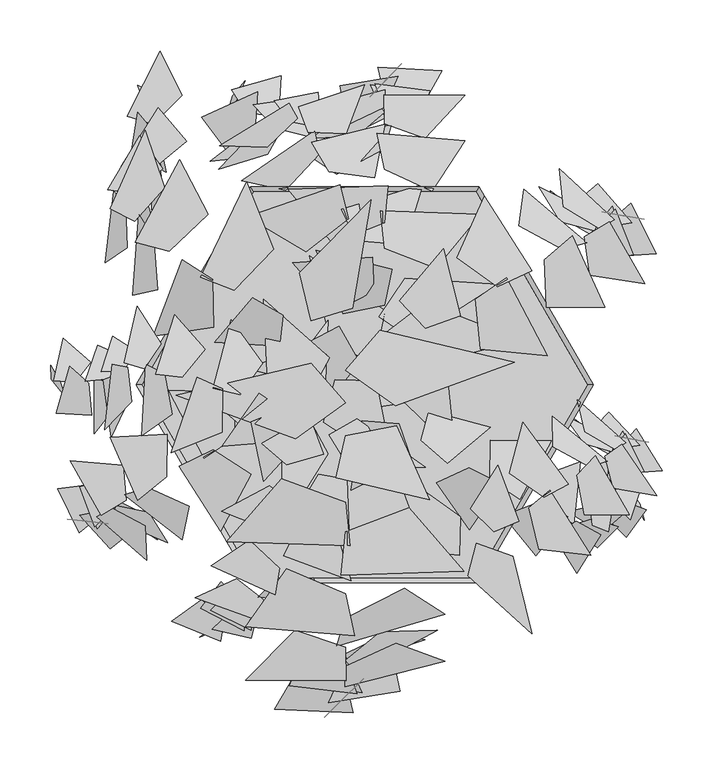
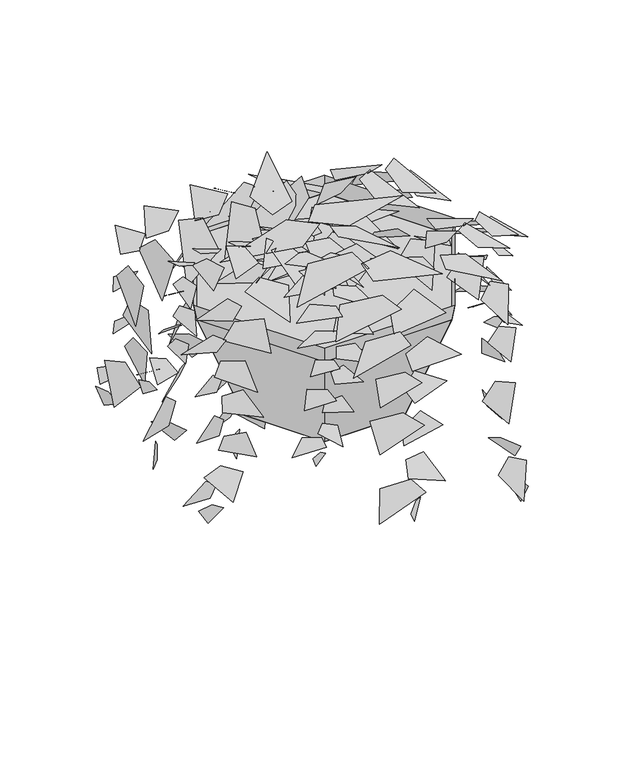
"""IFC4 building model written with IfcOpenShell, lengths in millimetres: geographic element geometry, 吊兰1 3D : 吊兰1 3D."""

import ifcopenshell
import ifcopenshell.guid

model = None  # the IFC model being written
_history = None  # IfcOwnerHistory: only IFC2X3 demands one
_inside = {}  # id of a spatial element -> (the spatial element, [elements in it])
_under = {}  # id of a project, library or spatial element -> (it, [spatial elements below it])
_declared = {}  # id of a project -> (the project, [libraries it declares])
_typed = {}  # id of a type object -> (the type object, [elements of that type])
_made_of = {}  # id of a material, layer set ... -> (it, [elements and type objects made of it])


def new_model(schema):
    """Start an empty IFC model of exactly this schema.

    Asked for "IFC4X3", IfcOpenShell would pick the latest addendum, in which some entities
    have other attributes; the version numbers below select the first issue.
    IFC2X3 requires an IfcOwnerHistory on every rooted entity: one is made here for all.
    """
    global model, _history
    if schema == "IFC4X3":
        model = ifcopenshell.file(schema_version=(4, 3, 0, 0))
    else:
        model = ifcopenshell.file(schema=schema)
    _inside.clear()
    _under.clear()
    _declared.clear()
    _typed.clear()
    _made_of.clear()
    _history = None
    if model.schema == "IFC2X3":
        org = make("IfcOrganization", Name="unknown")
        user = make(
            "IfcPersonAndOrganization",
            ThePerson=make("IfcPerson", FamilyName="unknown"),
            TheOrganization=org,
        )
        app = make(
            "IfcApplication",
            ApplicationDeveloper=org,
            Version="unknown",
            ApplicationFullName="unknown",
            ApplicationIdentifier="unknown",
        )
        _history = make(
            "IfcOwnerHistory",
            OwningUser=user,
            OwningApplication=app,
            ChangeAction="ADDED",
            CreationDate=0,
        )
    return model


def make(cls, **values):
    """One entity of the class cls with the attributes given. An attribute that is None is left unset."""
    return model.create_entity(
        cls, **{name: value for name, value in values.items() if value is not None}
    )


def rooted(cls, **values):
    """An entity with a GlobalId (a new one), such as an element, a storey or a relation."""
    return make(cls, GlobalId=ifcopenshell.guid.new(), OwnerHistory=_history, **values)


def si_unit(unit_type, name, prefix=None):
    """IfcSIUnit, for example si_unit("LENGTHUNIT", "METRE", prefix="MILLI")."""
    return make("IfcSIUnit", UnitType=unit_type, Prefix=prefix, Name=name)


def assignment(units):
    """IfcUnitAssignment: the units of a project."""
    return None if units is None else make("IfcUnitAssignment", Units=units)


def point(xyz):
    """IfcCartesianPoint."""
    return None if xyz is None else make("IfcCartesianPoint", Coordinates=xyz)


def direction(xyz):
    """IfcDirection."""
    return None if xyz is None else make("IfcDirection", DirectionRatios=xyz)


def frame(location, z_axis=None, x_axis=None):
    """IfcAxis2Placement3D, a coordinate frame: its origin and axes. An axis left out is left unset."""
    return make(
        "IfcAxis2Placement3D",
        Location=point(location),
        Axis=direction(z_axis),
        RefDirection=direction(x_axis),
    )


def origin():
    """The frame at (0, 0, 0) with its axes left unset."""
    return frame((0.0, 0.0, 0.0))


def place(relative_to, where):
    """IfcLocalPlacement: puts the frame where relative to a parent placement (None: the world)."""
    return make(
        "IfcLocalPlacement", PlacementRelTo=relative_to, RelativePlacement=where
    )


def context(
    kind, dimensions, precision=None, world=None, true_north=None, identifier=None
):
    """IfcGeometricRepresentationContext, for example the 3D "Model" context."""
    return make(
        "IfcGeometricRepresentationContext",
        ContextIdentifier=identifier,
        ContextType=kind,
        CoordinateSpaceDimension=dimensions,
        Precision=precision,
        WorldCoordinateSystem=world,
        TrueNorth=true_north,
    )


def project(units=None, contexts=None):
    """IfcProject with its units and contexts."""
    return rooted(
        "IfcProject",
        Name="project",
        RepresentationContexts=contexts,
        UnitsInContext=assignment(units),
    )


def spatial(cls, under=None, at=None, **own):
    """A site, building, storey or space (cls), placed at a placement, below another one or the project."""
    s = rooted(cls, ObjectPlacement=at, **own)
    if under is not None:
        _under.setdefault(under.id(), (under, []))[1].append(s)
    return s


def point_list(points):
    """IfcCartesianPointList2D or 3D."""
    cls = (
        "IfcCartesianPointList2D" if len(points[0]) == 2 else "IfcCartesianPointList3D"
    )
    return make(cls, CoordList=points)


def triangles(points, corners, closed=None, point_numbers=None):
    """IfcTriangulatedFaceSet: each triangle names its three corners, points numbered from 1."""
    return make(
        "IfcTriangulatedFaceSet",
        Coordinates=point_list(points),
        Closed=closed,
        CoordIndex=corners,
        PnIndex=point_numbers,
    )


def shape(context_of_items, identifier, shape_type, items):
    """IfcShapeRepresentation: the items that make up one representation, for example the "Body"."""
    return make(
        "IfcShapeRepresentation",
        ContextOfItems=context_of_items,
        RepresentationIdentifier=identifier,
        RepresentationType=shape_type,
        Items=items,
    )


def source(mapping_origin, context_of_items, identifier, shape_type, items):
    """IfcRepresentationMap: a shape defined once, which mapped items show again and again."""
    return make(
        "IfcRepresentationMap",
        MappingOrigin=mapping_origin,
        MappedRepresentation=shape(context_of_items, identifier, shape_type, items),
    )


def transform(
    local_origin,
    x_axis=None,
    y_axis=None,
    z_axis=None,
    scale=None,
    scale2=None,
    scale3=None,
    uniform=True,
):
    """IfcCartesianTransformationOperator3D, or its non-uniform kind. x_axis, y_axis, z_axis: its Axis1, 2, 3."""
    if uniform:
        return make(
            "IfcCartesianTransformationOperator3D",
            Axis1=direction(x_axis),
            Axis2=direction(y_axis),
            LocalOrigin=point(local_origin),
            Scale=scale,
            Axis3=direction(z_axis),
        )
    return make(
        "IfcCartesianTransformationOperator3DnonUniform",
        Axis1=direction(x_axis),
        Axis2=direction(y_axis),
        LocalOrigin=point(local_origin),
        Scale=scale,
        Axis3=direction(z_axis),
        Scale2=scale2,
        Scale3=scale3,
    )


def mapped(mapping_source, mapping_target):
    """IfcMappedItem: shows the shape of a source again, moved by a transform."""
    return make(
        "IfcMappedItem", MappingSource=mapping_source, MappingTarget=mapping_target
    )


def made_of(thing, what):
    """Note that an element or type object is made of a material, layer set ...; save() writes the relation."""
    if what is not None:
        _made_of.setdefault(what.id(), (what, []))[1].append(thing)
    return thing


def element(
    cls,
    number,
    at=None,
    inside=None,
    cuts=None,
    type_object=None,
    material=None,
    context=None,
    identifier="Body",
    shape_type=None,
    held_by="IfcProductDefinitionShape",
    body=None,
    shapes=None,
    **own,
):
    """One element of the class cls, such as IfcWall. Its Tag is "e" and its number.

    at: its placement. inside: the storey or other place that contains it. cuts: it is an
    opening in that element (IfcRelVoidsElement). A single representation is given by context,
    identifier, shape_type and body (its items); several are given by shapes. held_by: the class
    of the entity that holds the representations. save() writes the other relations.
    """
    e = rooted(cls, Tag="e%d" % number, ObjectPlacement=at, **own)
    if body is not None:
        shapes = [shape(context, identifier, shape_type, body)]
    if shapes is not None:
        e.Representation = make(held_by, Representations=shapes)
    if inside is not None:
        _inside.setdefault(inside.id(), (inside, []))[1].append(e)
    if cuts is not None:
        rooted(
            "IfcRelVoidsElement", RelatingBuildingElement=cuts, RelatedOpeningElement=e
        )
    if type_object is not None:
        _typed.setdefault(type_object.id(), (type_object, []))[1].append(e)
    return made_of(e, material)


def aggregate(whole, parts):
    """IfcRelAggregates: a whole, such as a stair, and the parts it consists of."""
    return rooted("IfcRelAggregates", RelatingObject=whole, RelatedObjects=parts)


def save(model, path):
    """Write the relations noted so far, then the file.

    IfcRelAggregates (storeys below a building ...), IfcRelContainedInSpatialStructure (elements
    in a storey), IfcRelDefinesByType, IfcRelAssociatesMaterial and IfcRelDeclares: one each for
    every whole, place, type object, material and project.
    """
    for whole, parts in _under.values():
        aggregate(whole, parts)
    for where, things in _inside.values():
        rooted(
            "IfcRelContainedInSpatialStructure",
            RelatedElements=things,
            RelatingStructure=where,
        )
    for kind, things in _typed.values():
        rooted("IfcRelDefinesByType", RelatedObjects=things, RelatingType=kind)
    for what, things in _made_of.values():
        rooted("IfcRelAssociatesMaterial", RelatedObjects=things, RelatingMaterial=what)
    for by, libraries in _declared.values():
        rooted("IfcRelDeclares", RelatingContext=by, RelatedDefinitions=libraries)
    model.write(path)


def geographic_element_80466ed5(model_context):
    return source(origin(), model_context, "Body", "Tessellation", [
        triangles([(24.2599631, 50.2389166, 267.3885118), (158.8119814, 43.5771957, 241.4721067), (63.9842803, 80.5561385, 262.1539112), (51.8116494, 16.5908296, 259.6649098)], [[2, 1, 3], [1, 2, 4]], closed=False),
        triangles([(24.2599631, 297.8005363, -268.7615384), (29.421192, 303.1911411, -320.0210549), (41.033937, 315.3199611, -277.6829052), (10.0666014, 282.9764229, -285.4699117)], [[2, 1, 3], [1, 2, 4]], closed=False),
        triangles([(24.2599631, 231.9569535, 214.9697455), (-55.0589394, 228.6345546, 153.0443647), (31.5375009, 255.6792337, 179.2892926), (-22.6770247, 206.5734557, 219.6875171)], [[2, 1, 3], [1, 2, 4]], closed=False),
        triangles([(24.2599631, 158.864213, 274.8400918), (-70.1672968, 192.1173976, 216.0915157), (27.7604104, 195.4893939, 266.9692786), (-26.4541175, 138.8656154, 253.3366078)], [[2, 1, 3], [1, 2, 4]], closed=False),
        triangles([(24.2599631, 264.165816, -46.7915162), (67.759595, 285.081963, -116.1540293), (10.9416377, 294.6632277, -58.048578), (59.3281056, 244.126505, -70.2157177)], [[2, 1, 3], [1, 2, 4]], closed=False),
        triangles([(24.2599631, 261.8733869, -98.1583799), (-39.0796095, 249.9470255, -144.0194432), (28.021089, 274.0554195, -130.6746818), (-11.170949, 243.7281827, -88.5725914)], [[2, 1, 3], [1, 2, 4]], closed=False),
        triangles([(24.2599631, 256.3557186, 184.0745019), (103.5788612, 284.2884068, 134.7257154), (23.7592397, 284.5728189, 176.8495614), (64.4201367, 242.1049715, 166.6250947)], [[2, 1, 3], [1, 2, 4]], closed=False),
        triangles([(24.2599631, 272.6144646, -176.3554237), (-19.2396687, 293.5306116, -245.7178687), (37.5782863, 303.1118581, -187.6124401), (-10.808177, 252.5751354, -199.7795935)], [[2, 1, 3], [1, 2, 4]], closed=False),
        triangles([(24.2599631, 267.4978982, 27.8713956), (-49.0186331, 242.2327798, -28.3965589), (15.3293536, 279.018525, -7.0362603), (-3.4487269, 243.3447214, 34.645076)], [[2, 1, 3], [1, 2, 4]], closed=False),
        triangles([(24.2599631, 269.8287879, 80.0999164), (68.9093068, 288.8053731, 27.7385957), (15.09185, 295.8068534, 72.1218514), (55.7527424, 253.3390059, 61.8973392)], [[2, 1, 3], [1, 2, 4]], closed=False),
        triangles([(24.2599631, 284.5377012, -220.1010275), (80.7781181, 308.5586732, -286.3811933), (18.0590539, 311.7768634, -231.558831), (58.7199441, 269.3090341, -241.7832614)], [[2, 1, 3], [1, 2, 4]], closed=False),
        triangles([(24.2599631, 78.0773745, 293.4450608), (-42.655931, 131.9096628, 243.778979), (31.5863215, 113.4699362, 307.6653411), (-16.5243434, 69.6009388, 254.3917215)], [[2, 1, 3], [1, 2, 4]], closed=False),
        triangles([(24.2599631, 134.2455576, 280.5096949), (118.6872231, 167.4987514, 221.7611369), (20.7595137, 170.8707476, 272.6388817), (74.9740392, 114.2469691, 259.0062109)], [[2, 1, 3], [1, 2, 4]], closed=False),
        triangles([(24.2599631, 272.3845186, 137.3668151), (-55.0589394, 268.475255, 75.5038306), (24.7606843, 289.6767225, 106.4353002), (-15.9002104, 253.1376919, 137.3668151)], [[2, 1, 3], [1, 2, 4]], closed=False),
        triangles([(24.2599631, 22.4004632, 241.3319627), (-110.2920597, 15.7387434, 215.4155758), (-15.4643586, 52.7176897, 236.0973621), (-3.291726, -11.2476238, 233.6083607)], [[2, 1, 3], [1, 2, 4]], closed=False),
        triangles([(24.2599631, 211.4250309, 240.9685219), (103.5788612, 239.3577373, 191.6196991), (16.9824243, 246.7201149, 235.447638), (71.1969487, 190.0963182, 221.8149854)], [[2, 1, 3], [1, 2, 4]], closed=False),
        triangles([(117.4295419, 194.4478695, 230.2862161), (-104.3239374, 189.6404413, 201.8188949), (114.6539755, 189.6404413, 201.8188949), (-107.0995129, 194.4478695, 230.2862161), (-104.3239374, -189.6404413, 201.8188949), (-219.3640267, 0.0, 230.2862161), (-107.0995129, -194.4478513, 230.2862161), (-213.8128939, 0.0, 201.8188949), (74.250873, 119.6602288, 0.0), (74.250873, -119.6602197, 0.0), (143.336736, 0.0, 0.0), (-63.920844, -119.6602197, 0.0), (-63.920844, 119.6602288, 0.0), (-133.006707, 0.0, 0.0), (114.6539755, -189.6404413, 201.8188949), (117.4295419, -194.4478513, 230.2862161), (229.6940648, 0.0, 230.2862161), (224.1429501, 0.0, 201.8188949)], [[2, 1, 3], [1, 2, 4], [6, 5, 7], [5, 6, 8], [10, 9, 11], [9, 10, 12], [9, 12, 13], [13, 12, 14], [15, 7, 5], [7, 15, 16], [15, 17, 16], [17, 15, 18], [3, 17, 18], [17, 3, 1], [6, 2, 8], [2, 6, 4], [11, 3, 18], [9, 3, 11], [10, 18, 15], [10, 11, 18], [5, 8, 12], [8, 14, 12], [8, 2, 14], [14, 2, 13], [13, 3, 9], [3, 13, 2], [10, 5, 12], [5, 10, 15]], closed=False),
        triangles([(114.6539755, 189.6404413, 201.8188949), (114.6539755, -189.6404413, 201.8188949), (224.1429501, 0.0, 201.8188949), (-104.3239374, -189.6404413, 201.8188949), (-104.3239374, 189.6404413, 201.8188949), (-213.8128939, 0.0, 201.8188949)], [[2, 1, 3], [1, 2, 4], [1, 4, 5], [5, 4, 6]], closed=False),
        triangles([(38.4629457, -38.2173666, 274.8093161), (-8.3769057, -103.3130525, 243.0681394), (51.1880501, -73.7424056, 267.4729179), (2.3179205, -35.2401682, 266.2751168)], [[2, 1, 3], [1, 2, 4]], closed=False),
        triangles([(270.0535744, -115.8882297, -184.5879699), (275.4567329, -116.9080984, -228.8560527), (279.6633802, -132.6685827, -193.4378657), (263.1453296, -99.6178021, -197.8721154)], [[2, 1, 3], [1, 2, 4]], closed=False),
        triangles([(191.25644, -124.3642385, 229.7241138), (216.7714705, -75.7812937, 182.3309674), (210.3505144, -136.9676571, 198.6269022), (184.91989, -87.469343, 237.1247885)], [[2, 1, 3], [1, 2, 4]], closed=False),
        triangles([(127.8423329, -93.0257081, 281.0728872), (188.2070622, -55.0235582, 237.4334724), (157.3925732, -112.4561718, 274.0445372), (128.4744437, -54.5941649, 266.2815299)], [[2, 1, 3], [1, 2, 4]], closed=False),
        triangles([(231.0691443, -118.0715358, 5.531341), (238.0634485, -145.4132262, -56.9785579), (261.057085, -125.3280605, -3.1957993), (204.578374, -124.4858517, -16.9964462)], [[2, 1, 3], [1, 2, 4]], closed=False),
        triangles([(231.7651048, -112.5413592, -38.4538846), (244.2966073, -69.4276572, -73.2159343), (242.2785255, -117.8139389, -66.5793391), (227.5174353, -85.7119467, -27.7094551)], [[2, 1, 3], [1, 2, 4]], closed=False),
        triangles([(212.9745911, -133.8934534, 203.2407376), (213.4054878, -185.2464326, 155.3182085), (236.8128526, -147.0855715, 197.0587203), (189.3517598, -146.3778203, 185.4615176)], [[2, 1, 3], [1, 2, 4]], closed=False),
        triangles([(244.5832541, -111.2196466, -105.4291207), (279.1493309, -92.8922587, -161.7609112), (266.1294861, -132.4587299, -116.0478766), (240.3200513, -80.8168784, -122.9763054)], [[2, 1, 3], [1, 2, 4]], closed=False),
        triangles([(230.0575782, -126.1097624, 69.4649823), (235.2421818, -70.237814, 26.5112747), (244.1673274, -124.1858973, 40.1936994), (218.5401308, -100.0976601, 77.2593921)], [[2, 1, 3], [1, 2, 4]], closed=False),
        triangles([(229.3499724, -131.7327023, 114.1880791), (233.5199759, -160.1626257, 66.1574898), (254.1230061, -139.1940474, 107.9790377), (206.6619132, -138.4863144, 96.3818077)], [[2, 1, 3], [1, 2, 4]], closed=False),
        triangles([(256.6410391, -113.429786, -142.9033413), (261.9195687, -149.4170244, -203.7015743), (281.6912179, -122.7804598, -152.3042845), (234.2301251, -122.0727269, -163.9015145)], [[2, 1, 3], [1, 2, 4]], closed=False),
        triangles([(60.1514792, -54.3258673, 297.0926034), (128.3434742, -41.8040117, 259.2549784), (86.356811, -77.0366495, 308.7114982), (68.0421495, -25.3541528, 266.554878)], [[2, 1, 3], [1, 2, 4]], closed=False),
        triangles([(107.214495, -81.2324781, 285.954675), (107.7274724, -142.3669551, 228.9040149), (138.983477, -96.9879117, 279.4234603), (75.7020153, -96.0442738, 263.9605233)], [[2, 1, 3], [1, 2, 4]], closed=False),
        triangles([(228.5740932, -137.898069, 163.2254838), (253.6010539, -89.0277781, 115.8864039), (244.2633426, -144.1429459, 136.6832177), (225.3983241, -107.2180377, 166.0982554)], [[2, 1, 3], [1, 2, 4]], closed=False),
        triangles([(16.7744156, -22.1088681, 252.5260468), (55.2189814, 54.0579921, 239.8948956), (54.6783713, -15.9284121, 250.8315827), (-1.9072565, 9.7941026, 247.9049263)], [[2, 1, 3], [1, 2, 4]], closed=False),
        triangles([(172.980339, -116.3452785, 252.0102535), (173.4112538, -167.6982486, 204.0877426), (204.7288008, -129.6553491, 247.7610942), (141.4473437, -128.7117021, 232.2981573)], [[2, 1, 3], [1, 2, 4]], closed=False),
        triangles([(40.2251837, 41.2979425, 281.4703557), (93.7744996, -64.9305434, 262.4798906), (84.3186178, 26.2653822, 277.6346523), (22.9064075, 3.2162593, 275.8108174)], [[2, 1, 3], [1, 2, 4]], closed=False),
        triangles([(257.1128127, 166.5180699, -111.3982149), (264.113421, 165.2991763, -148.95904), (279.8647851, 162.5566838, -117.9354067), (237.8611171, 169.8700092, -123.6414175)], [[2, 1, 3], [1, 2, 4]], closed=False),
        triangles([(199.4275256, 133.2134622, 243.0600549), (161.5087645, 192.1686481, 197.6837185), (223.4225362, 139.6491795, 216.9149211), (156.4731525, 156.2553243, 246.5170386)], [[2, 1, 3], [1, 2, 4]], closed=False),
        triangles([(135.3913089, 96.2421269, 286.9305602), (122.848052, 185.2473955, 243.8820251), (169.0234221, 112.0917318, 281.1631433), (95.4875763, 124.8951745, 271.1737095)], [[2, 1, 3], [1, 2, 4]], closed=False),
        triangles([(227.6455706, 149.5051549, 51.2522359), (265.1690251, 126.8313481, 0.4262923), (248.4860682, 175.1124218, 43.003507), (225.5668094, 112.5609891, 34.0879311)], [[2, 1, 3], [1, 2, 4]], closed=False),
        triangles([(225.6372085, 148.3456236, 13.6127229), (187.2331391, 190.733307, -19.9923798), (237.9698133, 151.6322416, -10.2138728), (194.1025599, 166.2528245, 20.6368081)], [[2, 1, 3], [1, 2, 4]], closed=False),
        triangles([(220.803183, 145.5547056, 220.4213023), (280.28291, 99.0477424, 184.2605553), (245.3030502, 160.2100792, 215.1271668), (226.0431793, 107.6458458, 207.6350914)], [[2, 1, 3], [1, 2, 4]], closed=False),
        triangles([(235.0473899, 153.7785859, -43.686832), (234.1730247, 197.6117752, -94.5127721), (267.6441829, 159.0233421, -51.93552), (202.0134142, 170.4504244, -60.8510959)], [[2, 1, 3], [1, 2, 4]], closed=False),
        triangles([(230.5648147, 151.1905716, 105.9621187), (176.0880527, 194.4292841, 64.7312778), (236.7163651, 163.8449046, 80.3832657), (197.1748651, 160.1555949, 110.9255966)], [[2, 1, 3], [1, 2, 4]], closed=False),
        triangles([(232.6068775, 152.3695604, 144.2330203), (268.9385262, 127.8358017, 105.8648136), (251.3197251, 172.5182306, 138.3870109), (232.0598542, 119.9540154, 130.8949355)], [[2, 1, 3], [1, 2, 4]], closed=False),
        triangles([(245.4932821, 159.8095405, -75.7418158), (291.4827169, 128.7541323, -124.3091638), (266.6205717, 178.3278142, -84.1375969), (247.360719, 125.7635717, -91.6296723)], [[2, 1, 3], [1, 2, 4]], closed=False),
        triangles([(64.6143291, 55.3790234, 300.5635217), (82.2426817, 133.7622931, 264.1702671), (98.8551488, 67.6804119, 310.9835615), (39.1876834, 82.2692698, 271.9468454)], [[2, 1, 3], [1, 2, 4]], closed=False),
        triangles([(113.8230215, 83.7896712, 291.0850123), (184.6322259, 28.4242575, 248.0364953), (144.3652343, 104.9911387, 285.3176136), (118.6854064, 34.9055002, 275.3281434)], [[2, 1, 3], [1, 2, 4]], closed=False),
        triangles([(234.8459487, 153.6622776, 186.1958114), (196.4130112, 212.3206158, 140.8652117), (250.2165585, 162.0261566, 163.5304979), (200.2588702, 174.627604, 186.1958114)], [[2, 1, 3], [1, 2, 4]], closed=False),
        triangles([(15.8360417, 27.2168661, 262.3772079), (-49.3858754, 126.7061741, 243.3867428), (24.86418, 72.9191774, 258.5415045), (-25.8030535, 31.2592043, 256.7176696)], [[2, 1, 3], [1, 2, 4]], closed=False),
        triangles([(181.4396155, 122.8281404, 262.1108724), (240.9193425, 76.3211863, 225.9501254), (209.1494612, 146.2442166, 258.0654071), (183.4696333, 76.1585781, 248.0759733)], [[2, 1, 3], [1, 2, 4]], closed=False),
        triangles([(-13.9299353, -17.8830325, 316.6156669), (-180.0435343, -10.1368483, 300.753045), (-62.9723054, -53.1356193, 313.4117563), (-47.9443619, 21.2426487, 311.8883028)], [[2, 1, 3], [1, 2, 4]], closed=False),
        triangles([(-13.9299353, -305.7454001, -11.5451279), (-20.3018245, -312.0135132, -42.9194733), (-34.638547, -326.1167948, -17.0056287), (3.5927333, -288.508062, -21.7718201)], [[2, 1, 3], [1, 2, 4]], closed=False),
        triangles([(-13.9299353, -229.1830676, 284.5317967), (83.9946278, -225.3198223, 246.6291866), (-22.9145488, -256.7671397, 262.6928863), (44.0169626, -199.667391, 287.4193567)], [[2, 1, 3], [1, 2, 4]], closed=False),
        triangles([(-13.9299353, -144.1915167, 321.176544), (102.6469322, -182.8580246, 285.2183827), (-18.251475, -186.7789517, 316.3590692), (48.6800364, -120.9373311, 308.0149564)], [[2, 1, 3], [1, 2, 4]], closed=False),
        triangles([(-13.9299353, -266.635251, 124.3158221), (-67.6331855, -290.9563683, 81.8612006), (2.5124409, -302.0973307, 117.4257358), (-57.2239326, -243.3337119, 109.978625)], [[2, 1, 3], [1, 2, 4]], closed=False),
        triangles([(-13.9299353, -263.9696434, 92.875799), (64.2670665, -250.1017581, 64.8056464), (-18.5733019, -278.1347853, 72.9735436), (29.8119317, -242.8705497, 98.7429372)], [[2, 1, 3], [1, 2, 4]], closed=False),
        triangles([(-13.9299353, -257.5537378, 265.6217773), (-111.8545007, -290.0335866, 235.4168986), (-13.311759, -290.3643259, 261.199609), (-63.5103948, -240.9830923, 254.9414881)], [[2, 1, 3], [1, 2, 4]], closed=False),
        triangles([(-13.9299353, -276.4592517, 45.0137904), (39.7733127, -300.7803507, 2.5592091), (-30.3723126, -311.9213313, 38.1236995), (29.3640643, -253.1576943, 30.6765909)], [[2, 1, 3], [1, 2, 4]], closed=False),
        triangles([(-13.9299353, -270.5097784, 170.014677), (76.5374703, -241.1317387, 135.5748188), (-2.9044926, -283.9058357, 148.6487846), (20.2783226, -242.4246649, 174.1606449)], [[2, 1, 3], [1, 2, 4]], closed=False),
        triangles([(-13.9299353, -273.2200962, 201.9821661), (-69.0525756, -295.2859005, 169.9333956), (-2.6112789, -303.427155, 197.099034), (-52.8099124, -254.0459395, 190.8408949)], [[2, 1, 3], [1, 2, 4]], closed=False),
        triangles([(-13.9299353, -290.3234672, 18.2384546), (-83.7054285, -318.2548837, -22.3295418), (-6.2744915, -321.9969518, 11.2255287), (-56.4731245, -272.6157181, 4.9674032)], [[2, 1, 3], [1, 2, 4]], closed=False),
        triangles([(-13.9299353, -50.2533279, 332.5640757), (68.6822766, -112.8490075, 302.1650046), (-22.974824, -91.4074838, 341.2678685), (36.42106, -40.3970119, 308.6607382)], [[2, 1, 3], [1, 2, 4]], closed=False),
        triangles([(-13.9299353, -115.5651753, 324.6467537), (-130.5068051, -154.2316651, 288.6885561), (-9.6083956, -158.1526103, 319.8292425), (-76.5399048, -92.3109897, 311.4851297)], [[2, 1, 3], [1, 2, 4]], closed=False),
        triangles([(-13.9299353, -276.1918807, 237.0334242), (83.9946278, -271.6462097, 199.1690203), (-14.5481105, -296.2990836, 218.1012404), (35.6505242, -253.8118332, 237.0334242)], [[2, 1, 3], [1, 2, 4]], closed=False),
        triangles([(-13.9299353, 14.4872618, 300.6672762), (152.1836705, 22.2334471, 284.8046544), (35.1124371, -20.7653273, 297.4633475), (20.0844935, 53.612943, 295.939894)], [[2, 1, 3], [1, 2, 4]], closed=False),
        triangles([(-13.9299353, -205.3087618, 300.4448153), (-111.8545007, -237.7886288, 270.2399365), (-4.9453195, -246.3495343, 297.065661), (-71.8768309, -180.5079319, 288.7215483)], [[2, 1, 3], [1, 2, 4]], closed=False),
        triangles([(-48.5601219, -8.9692711, 288.2841476), (-94.5697999, 84.200193, 272.6449496), (-90.4275927, 2.2078228, 285.125347), (-29.6974855, 26.4383662, 283.6233493)], [[2, 1, 3], [1, 2, 4]], closed=False),
        triangles([(-265.4477509, -134.1893928, -35.2546931), (-272.159169, -133.4714406, -66.1871119), (-287.2598097, -131.8560232, -40.6382717), (-246.9913919, -136.1637908, -45.3373035)], [[2, 1, 3], [1, 2, 4]], closed=False),
        triangles([(-207.7624819, -100.8847941, 256.6521576), (-174.2883442, -152.1416219, 219.2833812), (-231.3496505, -108.0268273, 235.1208411), (-167.4381991, -119.3711567, 259.4990587)], [[2, 1, 3], [1, 2, 4]], closed=False),
        triangles([(-143.7262471, -63.9134589, 292.7807845), (-136.4742279, -143.7540434, 257.3290604), (-177.162224, -80.1027959, 288.0311653), (-106.6642742, -87.6444141, 279.804578)], [[2, 1, 3], [1, 2, 4]], closed=False),
        triangles([(-235.9805088, -117.1764868, 98.6927404), (-271.0664668, -98.7245608, 56.8361066), (-257.5672907, -141.4911364, 91.8997049), (-231.9367149, -83.6358742, 84.557475)], [[2, 1, 3], [1, 2, 4]], closed=False),
        triangles([(-233.9721467, -116.0169464, 67.6955046), (-199.1172974, -152.2571853, 40.0207494), (-246.0940085, -119.6686131, 48.0735918), (-204.422842, -130.4853947, 73.4800398)], [[2, 1, 3], [1, 2, 4]], closed=False),
        triangles([(-229.1381394, -113.2260376, 238.0084737), (-284.1732067, -74.4174144, 208.2290051), (-253.6660572, -127.8328131, 233.6485836), (-232.1277462, -79.2149413, 227.4786295)], [[2, 1, 3], [1, 2, 4]], closed=False),
        triangles([(-243.3823281, -121.4499269, 20.5076713), (-244.9454594, -161.0612082, -21.3490012), (-275.2328186, -127.9873004, 13.7145971), (-212.3134033, -134.7181941, 6.3723684)], [[2, 1, 3], [1, 2, 4]], closed=False),
        triangles([(-238.8997347, -118.8619036, 143.7479845), (-188.5291719, -154.9885048, 109.793153), (-245.5517269, -130.6494744, 122.6830185), (-207.0624701, -125.1376288, 147.835553)], [[2, 1, 3], [1, 2, 4]], closed=False),
        triangles([(-240.9418157, -120.0408923, 175.2651741), (-274.7715458, -99.8405901, 143.6678477), (-260.1683856, -139.2997549, 170.4508059), (-238.6300927, -90.6818922, 164.2808882)], [[2, 1, 3], [1, 2, 4]], closed=False),
        triangles([(-253.8282203, -127.4808724, -5.8905539), (-296.6506428, -101.910867, -45.8871973), (-275.3029814, -145.3972934, -12.8047337), (-253.7646704, -96.7794306, -18.9746969)], [[2, 1, 3], [1, 2, 4]], closed=False),
        triangles([(-72.9492673, -23.0503486, 304.0079335), (-94.3272638, -94.9390633, 274.0370158), (-106.7795561, -36.0628015, 312.5891685), (-49.8079745, -45.9822542, 280.4412761)], [[2, 1, 3], [1, 2, 4]], closed=False),
        triangles([(-122.1579597, -51.4610031, 296.2021055), (-187.6759355, -5.2602746, 260.7503813), (-152.8963178, -72.3227294, 291.4524681), (-124.1785849, -7.4989109, 283.2258808)], [[2, 1, 3], [1, 2, 4]], closed=False),
        triangles([(-243.1808869, -121.3336186, 209.8227668), (-209.1925727, -172.2936077, 172.4916515), (-258.523446, -129.7460685, 191.1572273), (-210.8441616, -138.4011452, 209.8227668)], [[2, 1, 3], [1, 2, 4]], closed=False),
        triangles([(-24.1709788, 5.1118064, 272.5603618), (33.5113062, -81.318483, 256.9211637), (-35.4250724, -36.7350397, 269.4015793), (15.9242551, 3.7435104, 267.8995634)], [[2, 1, 3], [1, 2, 4]], closed=False),
        triangles([(-189.7745537, -90.4994724, 272.3410438), (-244.8096574, -51.6908538, 242.5616115), (-217.892187, -113.2092236, 269.0094884), (-189.1744632, -48.3854005, 260.7829011)], [[2, 1, 3], [1, 2, 4]], closed=False),
        triangles([(-47.7588581, 62.7239557, 295.9149137), (11.4063657, 181.4290057, 318.19613), (-59.0337922, 109.8756062, 303.7119305), (-6.9013093, 74.9248371, 299.2585141)], [[2, 1, 3], [1, 2, 4]], closed=False),
        triangles([(-209.5907679, 271.1982719, -95.0676983), (-206.9955229, 288.4365548, -130.5826907), (-217.8059096, 294.350329, -96.6955967), (-200.0780128, 256.6653836, -111.1972642)], [[2, 1, 3], [1, 2, 4]], closed=False),
        triangles([(-202.57112, 144.6294896, 255.1253976), (-222.8998755, 87.9166086, 186.3889864), (-217.0017436, 167.6029056, 231.1987331), (-198.3048652, 93.2996285, 244.6838293)], [[2, 1, 3], [1, 2, 4]], closed=False),
        triangles([(-144.3964006, 103.5981914, 299.5249768), (-203.0109188, 47.4945846, 227.8960822), (-174.5681418, 122.5598338, 294.3117775), (-143.5319185, 56.5847592, 268.923756)], [[2, 1, 3], [1, 2, 4]], closed=False),
        triangles([(-203.3509234, 211.7833666, 65.6812652), (-198.1403222, 271.8848943, 28.4954968), (-234.0766461, 214.5697699, 53.0142559), (-170.0199092, 239.0477453, 59.7554051)], [[2, 1, 3], [1, 2, 4]], closed=False),
        triangles([(-195.9039216, 221.5972298, 28.6457965), (-204.333567, 171.9392507, -23.502013), (-201.8066681, 236.3744346, 6.1222922), (-194.2160159, 181.9910354, 25.0953977)], [[2, 1, 3], [1, 2, 4]], closed=False),
        triangles([(-220.838101, 160.6005714, 232.4303985), (-210.4751797, 250.1250124, 220.4568016), (-245.1619615, 172.6968171, 226.6046094), (-191.3327435, 193.2665462, 232.2694163)], [[2, 1, 3], [1, 2, 4]], closed=False),
        triangles([(-197.1244503, 242.0955244, -27.9658325), (-224.5988271, 227.2553873, -91.5822733), (-217.8429713, 267.8268571, -32.5405442), (-190.1431359, 208.944114, -55.1993605)], [[2, 1, 3], [1, 2, 4]], closed=False),
        triangles([(-214.1753536, 197.5187031, 119.5132265), (-213.4700006, 136.2589067, 57.0520863), (-224.0101457, 201.603392, 91.4188203), (-203.9878758, 162.804107, 116.3770807)], [[2, 1, 3], [1, 2, 4]], closed=False),
        triangles([(-221.7472933, 187.5402061, 157.1699487), (-216.1885301, 244.3300173, 132.635218), (-247.2722069, 191.4527943, 148.2038535), (-193.4430071, 212.0225417, 153.8686785)], [[2, 1, 3], [1, 2, 4]], closed=False),
        triangles([(-203.0260705, 255.8729356, -59.732237), (-195.9896722, 327.758773, -90.7888897), (-228.1815844, 263.5595304, -70.3287922), (-174.3523664, 284.1292595, -64.6640081)], [[2, 1, 3], [1, 2, 4]], closed=False),
        triangles([(-75.0749324, 68.1649163, 314.267518), (-142.4716453, 41.9041373, 257.2168034), (-105.054407, 85.3350892, 326.1804173), (-78.7938097, 37.8643562, 273.8292523)], [[2, 1, 3], [1, 2, 4]], closed=False),
        triangles([(-123.2716635, 92.8003948, 304.0175623), (-110.9348529, 199.3771108, 289.7632906), (-156.0735948, 105.7314278, 296.677458), (-84.3013224, 133.1577334, 304.2305398)], [[2, 1, 3], [1, 2, 4]], closed=False),
        triangles([(-230.0496572, 176.5991406, 198.4593616), (-249.867143, 119.6440234, 129.7775164), (-241.8538785, 190.2333557, 176.0059719), (-228.1541878, 134.4873488, 186.5718059)], [[2, 1, 3], [1, 2, 4]], closed=False),
        triangles([(-20.4427861, 57.2829952, 277.5623094), (-62.3780557, -55.8196442, 218.088832), (-61.5660186, 35.9971442, 261.2225545), (-0.287187, 22.0175287, 264.1653255)], [[2, 1, 3], [1, 2, 4]], closed=False),
        triangles([(-187.1992022, 131.189585, 274.2235415), (-176.8362991, 220.714017, 262.2499628), (-220.4946263, 139.8575425, 267.4536059), (-148.7223538, 167.283848, 275.0066877)], [[2, 1, 3], [1, 2, 4]], closed=False),
        triangles([(-35.3498772, -68.4408352, 290.8146436), (-131.0758292, -27.3647791, 297.5505878), (-71.6593387, -78.6259057, 295.4211575), (-46.9033962, -37.71774, 289.5760928)], [[2, 1, 3], [1, 2, 4]], closed=False),
        triangles([(-140.3547687, -240.2170598, 80.6183895), (-149.3902546, -242.6058493, 60.2920003), (-157.4141743, -247.7869466, 80.0134391), (-127.8131105, -233.8415769, 71.0601066)], [[2, 1, 3], [1, 2, 4]], closed=False),
        triangles([(-85.8023027, -194.1109169, 278.1413074), (-33.5474663, -213.4092848, 241.7578633), (-99.7993408, -208.5775303, 265.4795985), (-45.6778396, -189.2934966, 272.6113216)], [[2, 1, 3], [1, 2, 4]], closed=False),
        triangles([(-62.4816104, -143.5147865, 299.3404677), (-8.5978315, -192.1895771, 264.1031382), (-74.9219576, -167.8905697, 298.3684158), (-23.0993667, -143.4763986, 282.6938275)], [[2, 1, 3], [1, 2, 4]], closed=False),
        triangles([(-114.4494458, -216.6956394, 171.0847425), (-156.0423104, -219.4371327, 149.0993203), (-113.6655365, -241.4028341, 166.1719973), (-136.0297965, -193.3592005, 165.0047539)], [[2, 1, 3], [1, 2, 4]], closed=False),
        triangles([(-117.8736372, -215.1742025, 149.6457168), (-73.4999104, -224.1705647, 121.6181035), (-126.1862113, -222.6141372, 137.2544855), (-87.3741998, -212.2324489, 148.0231596)], [[2, 1, 3], [1, 2, 4]], closed=False),
        triangles([(-94.4383944, -211.0135916, 266.535675), (-161.6566479, -208.8628326, 257.9556573), (-101.8462089, -230.6623014, 264.881143), (-120.6397111, -190.2895114, 263.9002436)], [[2, 1, 3], [1, 2, 4]], closed=False),
        triangles([(-126.7170564, -222.694601, 117.72024), (-106.623897, -249.0385417, 84.2075418), (-144.8195942, -240.1754199, 116.3368488), (-98.5679297, -218.3857615, 102.3472775)], [[2, 1, 3], [1, 2, 4]], closed=False),
        triangles([(-109.4723059, -218.907096, 202.2469029), (-55.4605592, -221.3927546, 167.915005), (-108.8038329, -229.3360016, 187.1482242), (-83.1349237, -209.7210288, 200.1796236)], [[2, 1, 3], [1, 2, 4]], closed=False),
        triangles([(-105.9906871, -220.4540764, 224.045536), (-146.5769997, -221.5221072, 209.1733515), (-106.7405141, -240.9074791, 220.817935), (-125.5340072, -200.5346891, 219.8370719)], [[2, 1, 3], [1, 2, 4]], closed=False),
        triangles([(-133.1732303, -230.9898432, 100.1560141), (-184.5483102, -232.3417956, 81.33041), (-136.6202492, -251.5142263, 95.9400469), (-155.4137514, -211.1414363, 94.9591384)], [[2, 1, 3], [1, 2, 4]], closed=False),
        triangles([(-40.4185858, -87.6510997, 303.0239456), (-10.582916, -143.075551, 276.231504), (-53.5330424, -110.1097943, 311.6680764), (-12.3863022, -92.9046217, 280.983594)], [[2, 1, 3], [1, 2, 4]], closed=False),
        triangles([(-55.7582154, -126.4911163, 300.4629646), (-135.7799389, -123.9306803, 290.2486171), (-63.2346486, -152.7662022, 298.5632986), (-88.2926394, -98.9358034, 297.2554387)], [[2, 1, 3], [1, 2, 4]], closed=False),
        triangles([(-102.1731966, -222.1502665, 247.9470931), (-49.7637639, -241.0429178, 211.5601789), (-109.3540628, -234.0050117, 236.0373367), (-68.7876027, -219.7418561, 241.6633741)], [[2, 1, 3], [1, 2, 4]], closed=False),
        triangles([(-30.2811663, -49.2305751, 278.6053598), (64.7985475, -81.160989, 249.6853045), (-10.2583185, -80.9696307, 272.685009), (-2.764155, -33.4567287, 270.0656558)], [[2, 1, 3], [1, 2, 4]], closed=False),
        triangles([(-78.5349138, -179.8870759, 287.9076263), (-145.7531583, -177.7363169, 279.3275904), (-82.8104795, -206.2645719, 286.4165473), (-107.8684703, -152.4341912, 285.1087056)], [[2, 1, 3], [1, 2, 4]], closed=False),
        triangles([(18.8485475, 66.6858369, 261.3560311), (135.2422446, 98.6711302, 220.0388402), (44.3797947, 104.746577, 252.2442508), (51.5141521, 44.6177435, 249.809225)], [[2, 1, 3], [1, 2, 4]], closed=False),
        triangles([(-121.2122416, 278.3727613, -225.6757599), (-124.9021962, 283.895462, -273.3895626), (-112.6432788, 298.5273451, -235.5763729), (-131.6261863, 260.979528, -239.6321028)], [[2, 1, 3], [1, 2, 4]], closed=False),
        triangles([(-39.4748207, 226.8430578, 217.9417116), (-116.1030149, 200.4889615, 171.0235544), (-44.4730803, 249.4158988, 184.788866), (-72.790656, 191.0931687, 227.6354695)], [[2, 1, 3], [1, 2, 4]], closed=False),
        triangles([(-10.9574128, 162.9653616, 271.1146651), (-110.7715726, 164.7447043, 230.0372851), (-19.294262, 196.2776633, 264.3955622), (-52.5276395, 130.5427222, 257.2950871)], [[2, 1, 3], [1, 2, 4]], closed=False),
        triangles([(-82.7360382, 251.6983539, -22.2040703), (-59.5960807, 281.6115171, -91.0943489), (-104.5137605, 274.757139, -30.0446414), (-49.3883326, 243.5961595, -48.8086396)], [[2, 1, 3], [1, 2, 4]], closed=False),
        triangles([(-88.7850512, 248.950066, -69.5589628), (-146.8804605, 219.7449446, -103.9681179), (-93.1817396, 260.3500606, -99.6548819), (-113.4360629, 222.9475289, -56.6675758)], [[2, 1, 3], [1, 2, 4]], closed=False),
        triangles([(-50.416849, 248.0131682, 190.1472054), (4.7275066, 294.6001684, 135.2711673), (-59.792703, 272.7527555, 184.3122236), (-13.4688136, 246.5670537, 168.5441636)], [[2, 1, 3], [1, 2, 4]], closed=False),
        triangles([(-102.0257583, 257.3661039, -141.2688117), (-155.1089553, 262.5499444, -198.9873998), (-100.4661515, 287.9962837, -152.5298613), (-130.12695, 229.3278444, -158.8670471)], [[2, 1, 3], [1, 2, 4]], closed=False),
        triangles([(-73.9436561, 255.6930592, 46.6274092), (-138.3247599, 211.7072629, 3.5570023), (-89.5844755, 262.8664041, 15.9418537), (-90.4933863, 226.5268162, 55.7777409)], [[2, 1, 3], [1, 2, 4]], closed=False),
        triangles([(-67.7931776, 258.4874381, 94.7766368), (-40.8793089, 287.2479827, 41.3400639), (-84.226654, 278.7704297, 89.3015168), (-37.9027691, 252.5847279, 73.5334885)], [[2, 1, 3], [1, 2, 4]], closed=False),
        triangles([(-111.1087522, 267.310773, -181.2275645), (-77.0405646, 303.7165269, -248.8688391), (-125.7536432, 289.5050579, -190.2538668), (-79.4297629, 263.3193561, -206.0219087)], [[2, 1, 3], [1, 2, 4]], closed=False),
        triangles([(14.3587802, 91.6981274, 286.0891326), (-65.9981154, 119.6449862, 250.3902579), (12.6040101, 125.315643, 299.1852446), (-24.0648987, 72.0540458, 255.1435833)], [[2, 1, 3], [1, 2, 4]], closed=False),
        triangles([(-3.2426587, 141.2476738, 275.6779222), (62.4053796, 196.7083965, 210.3493153), (-17.7132402, 172.5699898, 269.8578014), (44.0519441, 137.6557147, 248.8337395)], [[2, 1, 3], [1, 2, 4]], closed=False),
        triangles([(-61.0493759, 261.5514044, 147.5707799), (-137.503144, 234.6785534, 100.6943806), (-69.5438656, 276.5712725, 119.4889729), (-90.781768, 233.0950926, 152.2143373)], [[2, 1, 3], [1, 2, 4]], closed=False),
        triangles([(23.3383147, 41.6735464, 236.622966), (-96.0396411, -2.8332522, 229.8619869), (-20.7382304, 57.1512218, 237.7133245), (7.7258803, 3.9424695, 232.1521088)], [[2, 1, 3], [1, 2, 4]], closed=False),
        triangles([(-30.266957, 209.0281205, 241.3311633), (24.8773968, 255.6151206, 186.4551161), (-47.3634607, 238.1319945, 238.1241825), (14.4017236, 203.2177375, 217.1001024)], [[2, 1, 3], [1, 2, 4]], closed=False),
        triangles([(114.8801517, -155.7273768, 297.8234636), (169.094784, -244.2542044, 286.8760396), (150.6048697, -168.4626823, 295.6122977), (106.2627544, -187.2555033, 294.5609084)], [[2, 1, 3], [1, 2, 4]], closed=False),
        triangles([(266.0881732, -52.9665163, 71.3462992), (271.6163605, -54.0186232, 49.6935919), (284.0547728, -56.385857, 67.5777747), (250.8856673, -50.073229, 64.2884451)], [[2, 1, 3], [1, 2, 4]], closed=False),
        triangles([(225.8716055, -80.2976696, 275.681047), (189.4839646, -31.1199891, 249.5229416), (243.5133157, -75.0893347, 260.6091472), (190.0360567, -60.917162, 277.6738941)], [[2, 1, 3], [1, 2, 4]], closed=False),
        triangles([(181.2273283, -110.637878, 300.9711276), (160.635235, -36.648106, 276.1549098), (205.1138972, -97.6661952, 297.646385), (147.0447219, -86.6146804, 291.8877431)], [[2, 1, 3], [1, 2, 4]], closed=False),
        triangles([(245.5444417, -66.9280187, 165.1094713), (277.1624246, -85.9719599, 135.8098244), (258.4028684, -45.7798728, 160.3543655), (248.4949884, -97.5981397, 155.2147991)], [[2, 1, 3], [1, 2, 4]], closed=False),
        triangles([(244.1442547, -67.8795867, 143.4114316), (209.4231182, -32.4583613, 124.0390585), (253.2141044, -65.2202196, 129.6760963), (217.7138367, -52.8283434, 147.4605849)], [[2, 1, 3], [1, 2, 4]], closed=False),
        triangles([(240.7741116, -70.1699311, 262.630481), (292.1934475, -109.1320832, 241.7848783), (257.7919137, -58.1380892, 259.5785779), (249.4659865, -101.6828468, 255.2596009)], [[2, 1, 3], [1, 2, 4]], closed=False),
        triangles([(250.7047736, -63.4210653, 110.3799086), (244.6375204, -27.0128679, 81.0802526), (275.1013404, -59.2507484, 105.6247937), (223.2745983, -49.3872743, 100.4852364)], [[2, 1, 3], [1, 2, 4]], closed=False),
        triangles([(247.5796373, -65.5449, 196.6481712), (200.4060814, -29.3254788, 172.8798001), (250.7478669, -55.0705303, 181.9026868), (220.8246388, -57.9095512, 199.5094428)], [[2, 1, 3], [1, 2, 4]], closed=False),
        triangles([(249.0033149, -64.5773673, 218.7101785), (279.9346573, -85.1592188, 196.5920337), (260.8991186, -47.9504525, 215.3401444), (252.5731733, -91.4952147, 211.0211493)], [[2, 1, 3], [1, 2, 4]], closed=False),
        triangles([(257.9873777, -58.471817, 91.9011855), (297.1409472, -84.5247916, 63.9035122), (271.9387427, -43.212683, 87.0612466), (263.6127975, -86.7574406, 82.7422878)], [[2, 1, 3], [1, 2, 4]], closed=False),
        triangles([(131.8835924, -144.1718594, 308.8301319), (135.7780041, -79.1752363, 287.8504714), (156.6745392, -134.1504054, 314.83696), (109.0398378, -121.6949974, 292.3334463)], [[2, 1, 3], [1, 2, 4]], closed=False),
        triangles([(166.19051, -120.8568945, 303.3660396), (227.4040338, -167.2403914, 278.5498218), (187.0445241, -103.4229205, 300.041297), (175.9432577, -161.4826033, 294.2826732)], [[2, 1, 3], [1, 2, 4]], closed=False),
        triangles([(250.5643388, -63.5165037, 242.9005079), (213.8182533, -14.5824368, 216.7687454), (261.3431322, -56.6578017, 229.8346085), (221.4124845, -45.9081762, 242.9005079)], [[2, 1, 3], [1, 2, 4]], closed=False),
        triangles([(97.8767201, -167.2829033, 286.8168135), (35.5242851, -84.2865159, 275.8693713), (99.1868872, -129.3787217, 284.6056658), (65.39034, -163.6888822, 283.5542765)], [[2, 1, 3], [1, 2, 4]], closed=False),
        triangles([(213.3309465, -88.8202962, 286.6632982), (264.7502644, -127.7824528, 265.8176774), (231.736382, -69.5309939, 284.3312094), (220.6351519, -127.5906677, 278.5725675)], [[2, 1, 3], [1, 2, 4]], closed=False),
        triangles([(-62.3404581, -30.8654057, 287.9505743), (-31.0890499, 63.2664281, 255.4141336), (-74.6140003, 4.9571681, 284.8787959), (-34.441214, -19.6220604, 274.7541414)], [[2, 1, 3], [1, 2, 4]], closed=False),
        triangles([(-294.1081563, 3.1549179, 115.2024249), (-302.7829901, 5.651079, 94.7323626), (-303.2845947, 19.103912, 112.022014), (-289.2691529, -11.5459954, 108.1478319)], [[2, 1, 3], [1, 2, 4]], closed=False),
        triangles([(-191.321298, 11.0612934, 298.203564), (-214.1622185, -50.0434252, 285.1170444), (-210.020956, 20.3506292, 286.8215734), (-184.042073, -28.780404, 303.0422948)], [[2, 1, 3], [1, 2, 4]], closed=False),
        triangles([(-134.7631677, -3.8752441, 309.6623486), (-185.2644184, -66.7564994, 306.5101064), (-159.6568972, 7.233842, 312.265569), (-135.1200591, -46.4249597, 305.4830252)], [[2, 1, 3], [1, 2, 4]], closed=False),
        triangles([(-244.6331238, 5.9445585, 198.586752), (-257.4570322, 38.9991911, 167.5420082), (-269.5340567, 3.2522738, 201.3955377), (-226.1441361, 25.1641594, 180.2555853)], [[2, 1, 3], [1, 2, 4]], closed=False),
        triangles([(-249.2810959, 2.8297785, 177.5542422), (-260.8282654, -48.0591305, 166.9480946), (-260.5904529, 6.9119157, 166.0030941), (-243.7453328, -26.6968125, 183.8023165)], [[2, 1, 3], [1, 2, 4]], closed=False),
        triangles([(-211.5166132, 15.5049459, 289.9952169), (-218.7082709, 77.1102188, 262.6162558), (-231.5455688, 21.6995907, 292.0327924), (-195.0834593, 40.1129404, 274.2681427)], [[2, 1, 3], [1, 2, 4]], closed=False),
        triangles([(-265.9625995, 1.5754986, 147.9881599), (-298.1068402, -28.1224795, 130.506251), (-284.9482139, 18.0962428, 146.644392), (-263.0490782, -29.7942343, 140.5909643)], [[2, 1, 3], [1, 2, 4]], closed=False),
        triangles([(-237.8771772, 10.4719671, 229.1579965), (-243.8831514, -51.3720051, 213.621681), (-251.8469822, 5.1186119, 218.5107176), (-226.9103139, -15.0966644, 232.0371085)], [[2, 1, 3], [1, 2, 4]], closed=False),
        triangles([(-233.151212, 13.6389965, 250.543319), (-242.3601158, 47.8925845, 225.8156314), (-253.6844972, 12.9957184, 253.2437356), (-217.2223878, 31.409068, 235.4790678)], [[2, 1, 3], [1, 2, 4]], closed=False),
        triangles([(-279.2868771, 2.323205, 132.467205), (-290.9437055, 45.6821771, 101.1662813), (-300.4321343, 3.9562737, 133.524299), (-263.9700249, 22.3696216, 115.7596584)], [[2, 1, 3], [1, 2, 4]], closed=False),
        triangles([(-77.9885718, -22.7482458, 303.2162667), (-135.1755881, -60.2909965, 302.9702607), (-98.5362456, -8.0836374, 313.8860733), (-86.0344106, -56.1842296, 292.423448)], [[2, 1, 3], [1, 2, 4]], closed=False),
        triangles([(-117.4619073, -9.6265268, 307.6980062), (-126.0233942, 63.7130805, 275.1039928), (-143.9103565, -3.5671895, 311.3926208), (-95.2942015, 20.9839413, 287.7064031)], [[2, 1, 3], [1, 2, 4]], closed=False),
        triangles([(-227.9693699, 17.111543, 273.9916516), (-250.4066268, -44.1339022, 260.8290648), (-243.260951, 20.1730215, 264.4660702), (-223.8964172, -16.5726587, 276.9358941)], [[2, 1, 3], [1, 2, 4]], closed=False),
        triangles([(-46.6923444, -38.9825633, 272.6849), (-75.202064, -138.9556081, 282.100786), (-76.6093954, -60.4663401, 281.9988482), (-31.0301508, -67.4853112, 268.0788766)], [[2, 1, 3], [1, 2, 4]], closed=False),
        triangles([(-174.3266776, 7.3218988, 305.1110275), (-181.5183171, 68.9271699, 277.7320483), (-200.4326604, 10.447651, 310.109378), (-151.8165145, 34.9987812, 286.4231602)], [[2, 1, 3], [1, 2, 4]], closed=False),
    ])


if __name__ == "__main__":
    model = new_model("IFC4")
    model_context = context("Model", 3, world=origin())
    ifc_project = project(units=[si_unit("LENGTHUNIT", "METRE", prefix="MILLI")], contexts=[model_context])
    site = spatial("IfcSite", under=ifc_project)
    building = spatial("IfcBuilding", under=site)
    placement = place(None, origin())
    geographic_element_shape = geographic_element_80466ed5(model_context)
    element("IfcGeographicElement", 1, ObjectType="吊兰1 3D : 吊兰1 3D", at=placement, inside=building, context=model_context, shape_type="MappedRepresentation", body=[
        mapped(geographic_element_shape, transform((0.0, 0.0, 0.0), x_axis=(1.0, 0.0, 0.0), y_axis=(0.0, 1.0, 0.0), z_axis=(0.0, 0.0, 1.0))),
    ])
    save(model, "model.ifc")

# Revit data of these elements
# Project information
#   项目发布日期 = "出图日期"
#   项目状态 = "项目状态"
#   客户姓名 = "所有者"
#   项目地址 = "请在此处输入地址"
#   项目名称 = "项目名称"
#   项目编号 = "项目编号"
# Type "吊兰1 3D : 吊兰1 3D"
#   Height = 1000 mm
